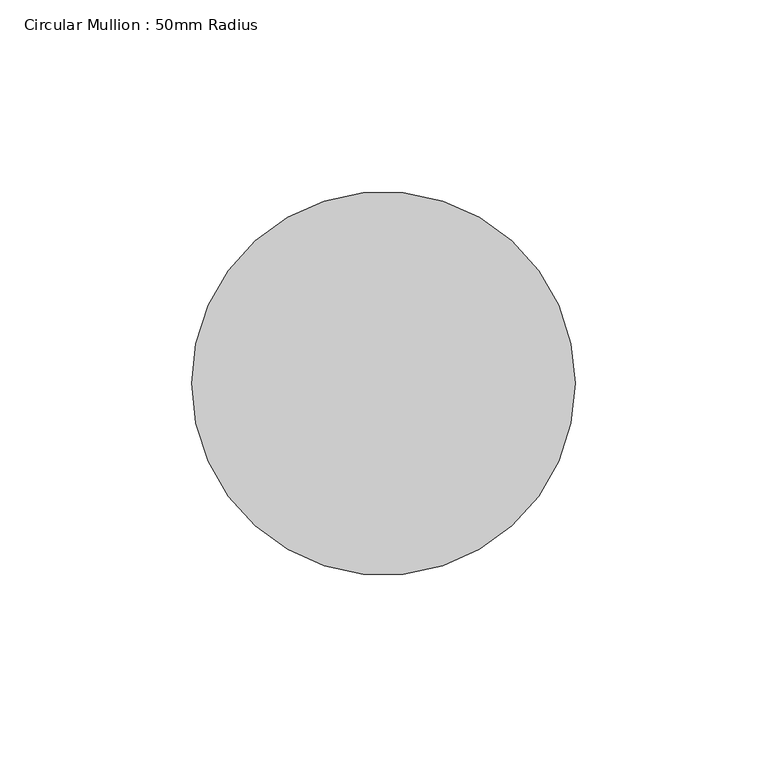
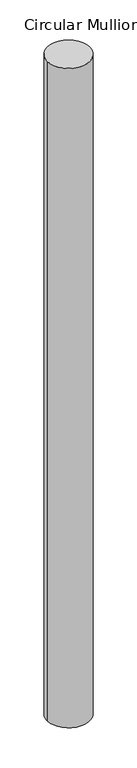
"""IFC4 building model written with IfcOpenShell, lengths in millimetres: member geometry, Circular Mullion : 50mm Radius."""

from ifc_helpers import new_model, si_unit, point, frame, origin, origin_2d, place, context, project, spatial, circle_curve, trimmed, segment, composite_curve, outline, extrude, source, transform, mapped, element, save


def circular_mullion_50mm_radius_efcf9aed(model_context):
    return source(origin(), model_context, "Body", "SweptSolid", [
        extrude(outline(composite_curve([segment(trimmed(circle_curve(origin_2d(), 50.0), [point((50.0, 0.0))], [point((-50.0, 0.0))], False, "CARTESIAN"), True, "CONTINUOUS"), segment(trimmed(circle_curve(origin_2d(), 50.0), [point((-50.0, 0.0))], [point((50.0, 0.0))], False, "CARTESIAN"), True, "CONTINUOUS")], self_intersect=False)), frame((0.0, 0.0, -1627.4592024), z_axis=(0.0, 0.0, 1.0), x_axis=(1.0, 0.0, 0.0)), (0.0, 0.0, 1.0), 1627.4592024),
    ])


if __name__ == "__main__":
    model = new_model("IFC4")
    model_context = context("Model", 3, world=origin())
    ifc_project = project(units=[si_unit("LENGTHUNIT", "METRE", prefix="MILLI")], contexts=[model_context])
    site = spatial("IfcSite", under=ifc_project)
    building = spatial("IfcBuilding", under=site)
    placement = place(None, origin())
    circular_mullion_50mm_radius_shape = circular_mullion_50mm_radius_efcf9aed(model_context)
    element("IfcMember", 1, ObjectType="Circular Mullion : 50mm Radius", at=placement, inside=building, context=model_context, shape_type="MappedRepresentation", body=[
        mapped(circular_mullion_50mm_radius_shape, transform((0.0, 0.0, 0.0), x_axis=(1.0, 0.0, 0.0), y_axis=(0.0, 1.0, 0.0), z_axis=(0.0, 0.0, 1.0))),
    ])
    save(model, "model.ifc")

# Revit data of these elements
# Type "Circular Mullion : 50mm Radius"
#   built-in parameter 1007350 = 0.164042 (stored number, unit not read)
# Element 1 (IfcMember, "Circular Mullion : 50mm Radius")
#   Materials on its faces: "Aluminium"
# Materials
#   "Aluminium": class "Metal", colour RGB 247 247 247, transparency 0, Description = "Aluminium 6061", Cost = 0
